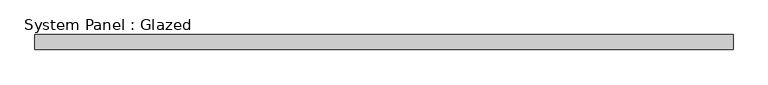
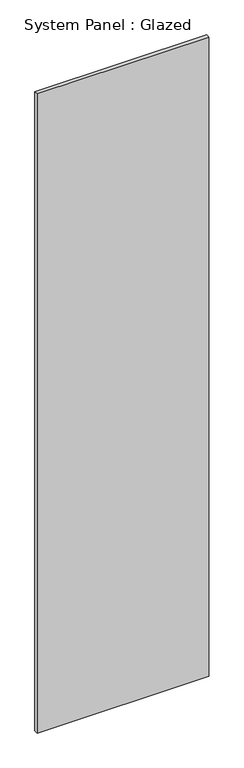
"""IFC4 building model written with IfcOpenShell, lengths in millimetres: plate geometry, System Panel : Glazed."""

import ifcopenshell
import ifcopenshell.guid

model = None  # the IFC model being written
_history = None  # IfcOwnerHistory: only IFC2X3 demands one
_inside = {}  # id of a spatial element -> (the spatial element, [elements in it])
_under = {}  # id of a project, library or spatial element -> (it, [spatial elements below it])
_declared = {}  # id of a project -> (the project, [libraries it declares])
_typed = {}  # id of a type object -> (the type object, [elements of that type])
_made_of = {}  # id of a material, layer set ... -> (it, [elements and type objects made of it])


def new_model(schema):
    """Start an empty IFC model of exactly this schema.

    Asked for "IFC4X3", IfcOpenShell would pick the latest addendum, in which some entities
    have other attributes; the version numbers below select the first issue.
    IFC2X3 requires an IfcOwnerHistory on every rooted entity: one is made here for all.
    """
    global model, _history
    if schema == "IFC4X3":
        model = ifcopenshell.file(schema_version=(4, 3, 0, 0))
    else:
        model = ifcopenshell.file(schema=schema)
    _inside.clear()
    _under.clear()
    _declared.clear()
    _typed.clear()
    _made_of.clear()
    _history = None
    if model.schema == "IFC2X3":
        org = make("IfcOrganization", Name="unknown")
        user = make(
            "IfcPersonAndOrganization",
            ThePerson=make("IfcPerson", FamilyName="unknown"),
            TheOrganization=org,
        )
        app = make(
            "IfcApplication",
            ApplicationDeveloper=org,
            Version="unknown",
            ApplicationFullName="unknown",
            ApplicationIdentifier="unknown",
        )
        _history = make(
            "IfcOwnerHistory",
            OwningUser=user,
            OwningApplication=app,
            ChangeAction="ADDED",
            CreationDate=0,
        )
    return model


def make(cls, **values):
    """One entity of the class cls with the attributes given. An attribute that is None is left unset."""
    return model.create_entity(
        cls, **{name: value for name, value in values.items() if value is not None}
    )


def rooted(cls, **values):
    """An entity with a GlobalId (a new one), such as an element, a storey or a relation."""
    return make(cls, GlobalId=ifcopenshell.guid.new(), OwnerHistory=_history, **values)


def si_unit(unit_type, name, prefix=None):
    """IfcSIUnit, for example si_unit("LENGTHUNIT", "METRE", prefix="MILLI")."""
    return make("IfcSIUnit", UnitType=unit_type, Prefix=prefix, Name=name)


def assignment(units):
    """IfcUnitAssignment: the units of a project."""
    return None if units is None else make("IfcUnitAssignment", Units=units)


def point(xyz):
    """IfcCartesianPoint."""
    return None if xyz is None else make("IfcCartesianPoint", Coordinates=xyz)


def direction(xyz):
    """IfcDirection."""
    return None if xyz is None else make("IfcDirection", DirectionRatios=xyz)


def frame(location, z_axis=None, x_axis=None):
    """IfcAxis2Placement3D, a coordinate frame: its origin and axes. An axis left out is left unset."""
    return make(
        "IfcAxis2Placement3D",
        Location=point(location),
        Axis=direction(z_axis),
        RefDirection=direction(x_axis),
    )


def origin():
    """The frame at (0, 0, 0) with its axes left unset."""
    return frame((0.0, 0.0, 0.0))


def origin_with_axes():
    """The frame at (0, 0, 0) with the z axis (0, 0, 1) and the x axis (1, 0, 0) written out."""
    return frame((0.0, 0.0, 0.0), z_axis=(0.0, 0.0, 1.0), x_axis=(1.0, 0.0, 0.0))


def place(relative_to, where):
    """IfcLocalPlacement: puts the frame where relative to a parent placement (None: the world)."""
    return make(
        "IfcLocalPlacement", PlacementRelTo=relative_to, RelativePlacement=where
    )


def context(
    kind, dimensions, precision=None, world=None, true_north=None, identifier=None
):
    """IfcGeometricRepresentationContext, for example the 3D "Model" context."""
    return make(
        "IfcGeometricRepresentationContext",
        ContextIdentifier=identifier,
        ContextType=kind,
        CoordinateSpaceDimension=dimensions,
        Precision=precision,
        WorldCoordinateSystem=world,
        TrueNorth=true_north,
    )


def project(units=None, contexts=None):
    """IfcProject with its units and contexts."""
    return rooted(
        "IfcProject",
        Name="project",
        RepresentationContexts=contexts,
        UnitsInContext=assignment(units),
    )


def spatial(cls, under=None, at=None, **own):
    """A site, building, storey or space (cls), placed at a placement, below another one or the project."""
    s = rooted(cls, ObjectPlacement=at, **own)
    if under is not None:
        _under.setdefault(under.id(), (under, []))[1].append(s)
    return s


def polyline(points):
    """IfcPolyline through the points."""
    return make("IfcPolyline", Points=[point(p) for p in points])


def outline(outer, holes=None, kind="AREA"):
    """IfcArbitraryClosedProfileDef: a profile drawn as a closed curve; with holes, ...WithVoids."""
    if holes is None:
        return make("IfcArbitraryClosedProfileDef", ProfileType=kind, OuterCurve=outer)
    return make(
        "IfcArbitraryProfileDefWithVoids",
        ProfileType=kind,
        OuterCurve=outer,
        InnerCurves=holes,
    )


def extrude(swept, where, along, depth):
    """IfcExtrudedAreaSolid: the profile swept, set in the frame where, extruded along a direction by depth."""
    return make(
        "IfcExtrudedAreaSolid",
        SweptArea=swept,
        Position=where,
        ExtrudedDirection=direction(along),
        Depth=depth,
    )


def shape(context_of_items, identifier, shape_type, items):
    """IfcShapeRepresentation: the items that make up one representation, for example the "Body"."""
    return make(
        "IfcShapeRepresentation",
        ContextOfItems=context_of_items,
        RepresentationIdentifier=identifier,
        RepresentationType=shape_type,
        Items=items,
    )


def source(mapping_origin, context_of_items, identifier, shape_type, items):
    """IfcRepresentationMap: a shape defined once, which mapped items show again and again."""
    return make(
        "IfcRepresentationMap",
        MappingOrigin=mapping_origin,
        MappedRepresentation=shape(context_of_items, identifier, shape_type, items),
    )


def transform(
    local_origin,
    x_axis=None,
    y_axis=None,
    z_axis=None,
    scale=None,
    scale2=None,
    scale3=None,
    uniform=True,
):
    """IfcCartesianTransformationOperator3D, or its non-uniform kind. x_axis, y_axis, z_axis: its Axis1, 2, 3."""
    if uniform:
        return make(
            "IfcCartesianTransformationOperator3D",
            Axis1=direction(x_axis),
            Axis2=direction(y_axis),
            LocalOrigin=point(local_origin),
            Scale=scale,
            Axis3=direction(z_axis),
        )
    return make(
        "IfcCartesianTransformationOperator3DnonUniform",
        Axis1=direction(x_axis),
        Axis2=direction(y_axis),
        LocalOrigin=point(local_origin),
        Scale=scale,
        Axis3=direction(z_axis),
        Scale2=scale2,
        Scale3=scale3,
    )


def mapped(mapping_source, mapping_target):
    """IfcMappedItem: shows the shape of a source again, moved by a transform."""
    return make(
        "IfcMappedItem", MappingSource=mapping_source, MappingTarget=mapping_target
    )


def made_of(thing, what):
    """Note that an element or type object is made of a material, layer set ...; save() writes the relation."""
    if what is not None:
        _made_of.setdefault(what.id(), (what, []))[1].append(thing)
    return thing


def element(
    cls,
    number,
    at=None,
    inside=None,
    cuts=None,
    type_object=None,
    material=None,
    context=None,
    identifier="Body",
    shape_type=None,
    held_by="IfcProductDefinitionShape",
    body=None,
    shapes=None,
    **own,
):
    """One element of the class cls, such as IfcWall. Its Tag is "e" and its number.

    at: its placement. inside: the storey or other place that contains it. cuts: it is an
    opening in that element (IfcRelVoidsElement). A single representation is given by context,
    identifier, shape_type and body (its items); several are given by shapes. held_by: the class
    of the entity that holds the representations. save() writes the other relations.
    """
    e = rooted(cls, Tag="e%d" % number, ObjectPlacement=at, **own)
    if body is not None:
        shapes = [shape(context, identifier, shape_type, body)]
    if shapes is not None:
        e.Representation = make(held_by, Representations=shapes)
    if inside is not None:
        _inside.setdefault(inside.id(), (inside, []))[1].append(e)
    if cuts is not None:
        rooted(
            "IfcRelVoidsElement", RelatingBuildingElement=cuts, RelatedOpeningElement=e
        )
    if type_object is not None:
        _typed.setdefault(type_object.id(), (type_object, []))[1].append(e)
    return made_of(e, material)


def aggregate(whole, parts):
    """IfcRelAggregates: a whole, such as a stair, and the parts it consists of."""
    return rooted("IfcRelAggregates", RelatingObject=whole, RelatedObjects=parts)


def save(model, path):
    """Write the relations noted so far, then the file.

    IfcRelAggregates (storeys below a building ...), IfcRelContainedInSpatialStructure (elements
    in a storey), IfcRelDefinesByType, IfcRelAssociatesMaterial and IfcRelDeclares: one each for
    every whole, place, type object, material and project.
    """
    for whole, parts in _under.values():
        aggregate(whole, parts)
    for where, things in _inside.values():
        rooted(
            "IfcRelContainedInSpatialStructure",
            RelatedElements=things,
            RelatingStructure=where,
        )
    for kind, things in _typed.values():
        rooted("IfcRelDefinesByType", RelatedObjects=things, RelatingType=kind)
    for what, things in _made_of.values():
        rooted("IfcRelAssociatesMaterial", RelatedObjects=things, RelatingMaterial=what)
    for by, libraries in _declared.values():
        rooted("IfcRelDeclares", RelatingContext=by, RelatedDefinitions=libraries)
    model.write(path)


def system_panel_glazed_38880ecf(model_context):
    return source(origin(), model_context, "Body", "SweptSolid", [
        extrude(outline(polyline([(587.8744819, 19.05), (-587.8744819, 19.05), (-587.8744819, 44.45), (587.8744819, 44.45), (587.8744819, 19.05)])), origin_with_axes(), (0.0, 0.0, 1.0), 4629.15),
    ])


if __name__ == "__main__":
    model = new_model("IFC4")
    model_context = context("Model", 3, world=origin())
    ifc_project = project(units=[si_unit("LENGTHUNIT", "METRE", prefix="MILLI")], contexts=[model_context])
    site = spatial("IfcSite", under=ifc_project)
    building = spatial("IfcBuilding", under=site)
    placement = place(None, origin())
    system_panel_glazed_shape = system_panel_glazed_38880ecf(model_context)
    element("IfcPlate", 1, ObjectType="System Panel : Glazed", at=placement, inside=building, context=model_context, shape_type="MappedRepresentation", body=[
        mapped(system_panel_glazed_shape, transform((0.0, 0.0, 0.0), x_axis=(1.0, 0.0, 0.0), y_axis=(0.0, 1.0, 0.0), z_axis=(0.0, 0.0, 1.0))),
    ])
    save(model, "model.ifc")

# Revit data of these elements
# Type "System Panel : Glazed"
#   Construction Type Id = "GSP4R"
#   Analytic Construction = "1/8 in Pilkington single glazing"
#   Visual Light Transmittance = 0.9
#   Solar Heat Gain Coefficient = 0.86
#   Heat Transfer Coefficient (U) = 1.18115 BTU/(h·ft²·°F)
#   Define Thermal Properties by = 1
# Element 1 (IfcPlate, "System Panel : Glazed")
#   Materials on its faces: "Glass"
# Materials
#   "Glass": class "Glass", colour RGB 0 128 192, transparency 0.75, Description = "Soda Lime Glass", Cost = 0
